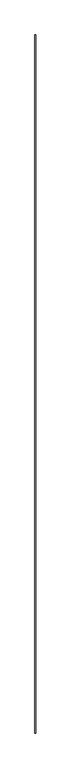
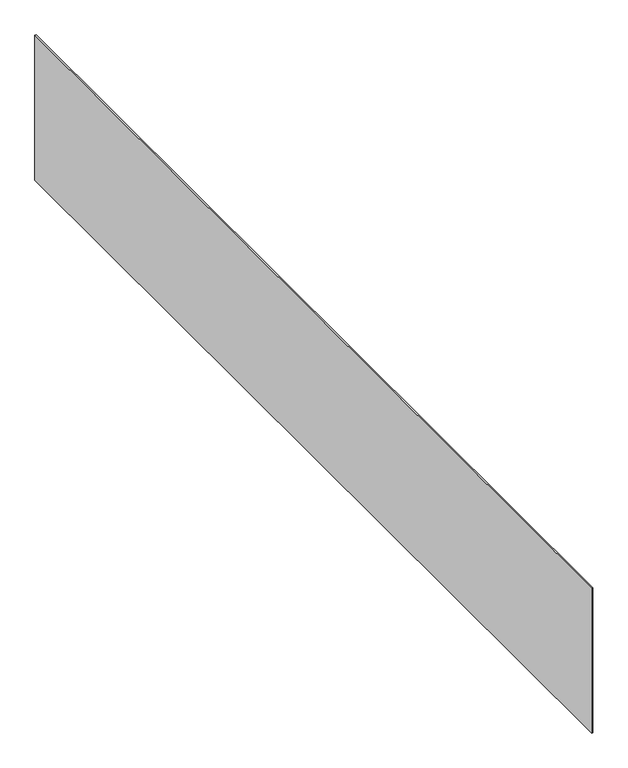
"""IFC4 building model written with IfcOpenShell, lengths in millimetres: proxy geometry, Panel:Panel:300402:Panel:300402 : Panel:Panel:300402:300124:Panel:300402:Panel:300402 : Panel:Panel:300402:300124 : Panel:Panel:300402:Panel:300402 : Panel:Panel:300402:300124:26 : Panel:Panel:300402:Panel:300402 : Panel:Panel:300402:300124:Panel:300402:Panel:300402 : Panel:Panel:300402:300124 : Panel:Panel:300402:Panel:300402 : Panel:Panel:300402:300124:300083."""

from ifc_helpers import new_model, si_unit, frame, origin, place, context, project, spatial, polyline, outline, extrude, source, transform, mapped, element, save


def generic_models_e11fa6b0(model_context):
    return source(origin(), model_context, "Body", "SweptSolid", [
        extrude(outline(polyline([(560264.0617239, -572944.1405465), (560264.0617239, -578718.1163841), (560256.1242239, -578718.1163841), (560256.1242239, -572944.1405465), (560264.0617239, -572944.1405465)])), frame((0.0, 0.0, 5217.8970827), z_axis=(0.0, 0.0, 1.0), x_axis=(1.0, 0.0, 0.0)), (0.0, 0.0, 1.0), 916.2029173),
    ])


if __name__ == "__main__":
    model = new_model("IFC4")
    model_context = context("Model", 3, world=origin())
    ifc_project = project(units=[si_unit("LENGTHUNIT", "METRE", prefix="MILLI")], contexts=[model_context])
    site = spatial("IfcSite", under=ifc_project)
    building = spatial("IfcBuilding", under=site)
    placement = place(None, origin())
    generic_models_shape = generic_models_e11fa6b0(model_context)
    element("IfcBuildingElementProxy", 1, Name="Panel:Panel:300402:Panel:300402 : Panel:Panel:300402:300124:Panel:300402:Panel:300402 : Panel:Panel:300402:300124 : Panel:Panel:300402:Panel:300402 : Panel:Panel:300402:300124:26 : Panel:Panel:300402:Panel:300402 : Panel:Panel:300402:300124:Panel:300402:Panel:300402 : Panel:Panel:300402:300124 : Panel:Panel:300402:Panel:300402 : Panel:Panel:300402:300124:300083", ObjectType="Panel:Panel:300402:Panel:300402 : Panel:Panel:300402:300124:Panel:300402:Panel:300402 : Panel:Panel:300402:300124 : Panel:Panel:300402:Panel:300402 : Panel:Panel:300402:300124:26 : Panel:Panel:300402:Panel:300402 : Panel:Panel:300402:300124:Panel:300402:Panel:300402 : Panel:Panel:300402:300124 : Panel:Panel:300402:Panel:300402 : Panel:Panel:300402:300124:300083", at=placement, inside=building, context=model_context, shape_type="MappedRepresentation", body=[
        mapped(generic_models_shape, transform((0.0, 0.0, 0.0), x_axis=(1.0, 0.0, 0.0), y_axis=(0.0, 1.0, 0.0), z_axis=(0.0, 0.0, 1.0))),
    ])
    save(model, "model.ifc")

# Revit data of these elements
# Type "Panel:Panel:300402:Panel:300402 : Panel:Panel:300402:300124:Panel:300402:Panel:300402 : Panel:Panel:300402:300124 : Panel:Panel:300402:Panel:300402 : Panel:Panel:300402:300124:26 : Panel:Panel:300402:Panel:300402 : Panel:Panel:300402:300124:Panel:300402:Panel:300402 : Panel:Panel:300402:300124 : Panel:Panel:300402:Panel:300402 : Panel:Panel:300402:300124:300083"
#   NameOverride = "Panel:Panel:300402:Panel:300402 : Panel:Panel:300402:300124:Panel:300402:Panel:300402 : Panel:Panel:300402:300124 : Panel:Panel:300402:Panel:300402 : Panel:Panel:300402:300124:300083"
#   ObjectTypeOverride = "Panel:300402:Panel:300402 : Panel:Panel:300402:300124 : Panel:Panel:300402:Panel:300402 : Panel:Panel:300402:300124"
#   Reference = "Panel"
#   Tag = "300083"
# Element 1 (IfcBuildingElementProxy, "Panel:Panel:300402:Panel:300402 : Panel:Panel:300402:300124:Panel:300402:Panel:300402 : Panel:Panel:300402:300124 : Panel:Panel:300402:Panel:300402 : Panel:Panel:300402:300124:26 : Panel:Panel:300402:Panel:300402 : Panel:Panel:300402:300124:Panel:300402:Panel:300402 : Panel:Panel:300402:300124 : Panel:Panel:300402:Panel:300402 : Panel:Panel:300402:300124:300083")
#   Materials on its faces: "5/16\" PHENOLIC RESIN PANELS (CLASS A FLAME SPREAD) - EXPOSED FASTENERS"
# Materials
#   "5/16\" PHENOLIC RESIN PANELS (CLASS A FLAME SPREAD) - EXPOSED FASTENERS": class "Unassigned", colour RGB 64 64 64, transparency 0, Keynote = "M07420000.01", Cost = 0
